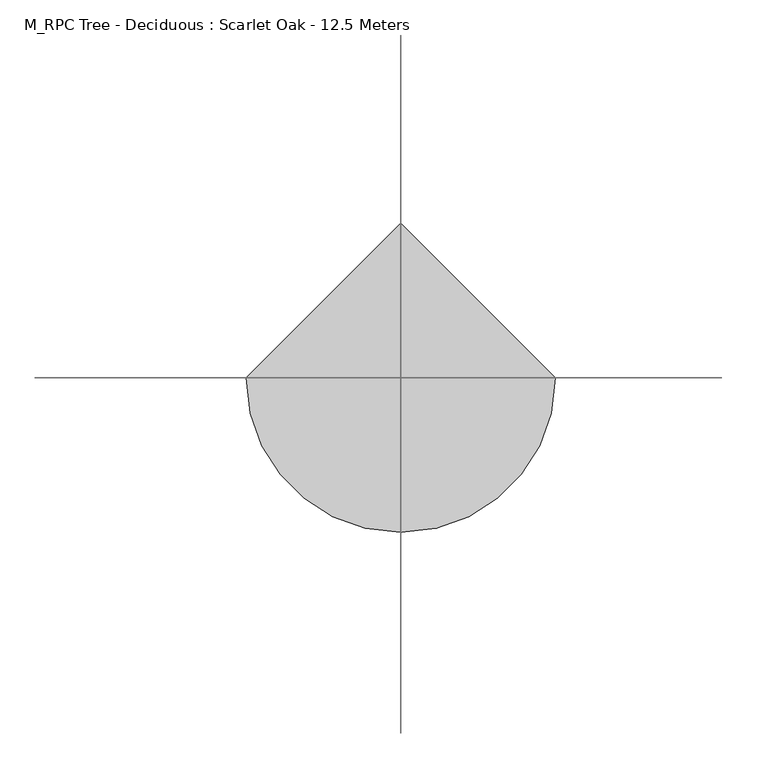
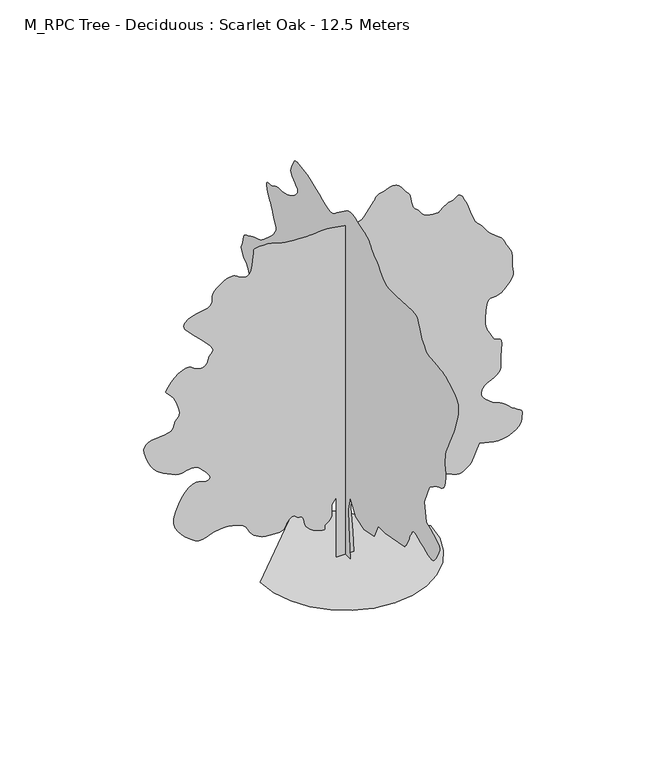
"""IFC4 building model written with IfcOpenShell, lengths in millimetres: geographic element geometry, M_RPC Tree - Deciduous : Scarlet Oak - 12.5 Meters."""

from ifc_helpers import new_model, si_unit, origin, place, context, project, spatial, triangles, source, transform, mapped, element, save


def m_rpc_tree_deciduous_scarlet_oak_12_5_meters_13b38d7d(model_context):
    return source(origin(), model_context, "Body", "Tessellation", [
        triangles([(0.0172504, 306.0074844, 0.0), (0.0172504, -293.5650026, 0.0), (0.0172504, -196.8600042, 1141.1199549), (0.0172504, -177.5184886, 1682.6674953), (0.0172504, -293.5650026, 2185.5349113), (0.0172504, -603.0224945, 1682.6674953), (0.0172504, -1105.8875124, 1527.9400211), (0.0172504, -1686.1174301, 1663.3275421), (0.0172504, -1918.2099495, 2146.8525341), (0.0172504, -2324.3725124, 2146.8525341), (0.0172504, -3446.1498253, 2359.6049549), (0.0172504, -3487.4249222, 2409.394939), (0.0172504, -3527.7000801, 2459.5225479), (0.0172504, -3565.9250725, 2510.3249702), (0.0172504, -3601.0999603, 2562.1500046), (0.0172504, -3632.2248047, 2615.3249565), (0.0172504, -3658.2749588, 2670.2000954), (0.0172504, -3678.2499023, 2727.0748215), (0.0172504, -3697.649881, 2785.6750237), (0.0172504, -3722.1248405, 2845.2748741), (0.0172504, -3750.8248329, 2905.7249634), (0.0172504, -3782.89991, 2966.8500114), (0.0172504, -3817.5248314, 3028.475029), (0.0172504, -3853.8249413, 3090.4500252), (0.0172504, -3890.9999977, 3152.5750122), (0.0172504, -3908.7000801, 3172.6499496), (0.0172504, -3933.1750397, 3188.8498329), (0.0172504, -3971.1750458, 3197.2499016), (0.0172504, -4029.4749756, 3193.9748108), (0.0172504, -4114.8499969, 3175.1500877), (0.0172504, -4234.0499886, 3136.8498093), (0.0172504, -4393.8498276, 3075.2250824), (0.0172504, -4562.5749939, 3002.6998581), (0.0172504, -4706.2499451, 2937.9750298), (0.0172504, -4828.2750549, 2886.4249786), (0.0172504, -4932.0251175, 2853.4999535), (0.0172504, -5020.8999252, 2844.5999153), (0.0172504, -5098.249855, 2865.1248253), (0.0172504, -5167.4996979, 2920.4999336), (0.0172504, -5237.3750839, 3007.7248421), (0.0172504, -5309.5997452, 3113.9000473), (0.0172504, -5377.0996948, 3229.5499649), (0.0172504, -5432.7497864, 3345.1998825), (0.0172504, -5469.4498718, 3451.3750877), (0.0172504, -5480.1248016, 3538.6249947), (0.0172504, -5457.6250122, 3597.424894), (0.0172504, -5402.6498795, 3641.6998077), (0.0172504, -5323.3000717, 3691.0249947), (0.0172504, -5223.6747574, 3744.5999222), (0.0172504, -5107.774855, 3801.5499344), (0.0172504, -4979.7251129, 3861.0500816), (0.0172504, -4843.5499947, 3922.224836), (0.0172504, -4703.3248329, 3984.2498291), (0.0172504, -4587.2749397, 4641.8498062), (0.0172504, -4877.3749649, 5318.7747665), (0.0172504, -4886.5249878, 5331.7001404), (0.0172504, -4900.7247025, 5347.4747589), (0.0172504, -4925.0999588, 5369.0251877), (0.0172504, -4964.6748688, 5399.20009), (0.0172504, -5024.5497025, 5440.8498734), (0.0172504, -5109.8247299, 5496.8999405), (0.0172504, -5225.5246445, 5570.225116), (0.0172504, -5351.0501221, 5636.6501312), (0.0172504, -5462.3497238, 5680.0498077), (0.0172504, -5559.4501923, 5715.3499786), (0.0172504, -5642.3497833, 5757.424736), (0.0172504, -5711.0246613, 5821.1499161), (0.0172504, -5765.4998245, 5921.4001923), (0.0172504, -5805.7496933, 6073.0746552), (0.0172504, -5829.0500153, 6222.0498642), (0.0172504, -5835.7501877, 6317.5748474), (0.0172504, -5830.6249191, 6379.6001312), (0.0172504, -5818.3750854, 6428.1000778), (0.0172504, -5803.7748138, 6483.0246323), (0.0172504, -5791.5499786, 6564.3249023), (0.0172504, -5786.4247101, 6691.9996674), (0.0172504, -5788.2251816, 6832.849791), (0.0172504, -5796.1246994, 6949.6746368), (0.0172504, -5813.8247818, 7056.3751007), (0.0172504, -5845.0496201, 7166.7747574), (0.0172504, -5893.550148, 7294.7750839), (0.0172504, -5963.0249771, 7454.2496521), (0.0172504, -6057.1750443, 7659.049942), (0.0172504, -6146.5748199, 7844.1746887), (0.0172504, -6206.1746704, 7955.8748474), (0.0172504, -6246.4751175, 8024.9497009), (0.0172504, -6277.9999374, 8082.1746964), (0.0172504, -6311.2246536, 8158.3496979), (0.0172504, -6356.599791, 8284.2751511), (0.0172504, -6424.6747055, 8490.6997604), (0.0172504, -6498.0248795, 8729.4997192), (0.0172504, -6547.3747742, 8935.1499573), (0.0172504, -6565.2498459, 9112.3746048), (0.0172504, -6544.199968, 9265.925116), (0.0172504, -6476.8250107, 9400.5250397), (0.0172504, -6355.6498489, 9520.8996689), (0.0172504, -6173.2249374, 9631.8248749), (0.0172504, -5996.2246948, 9723.0001236), (0.0172504, -5879.7998245, 9785.7747803), (0.0172504, -5799.2250916, 9827.2001587), (0.0172504, -5729.799678, 9854.4496582), (0.0172504, -5646.85009, 9874.575174), (0.0172504, -5525.6749283, 9894.699527), (0.0172504, -5341.575119, 9921.9501892), (0.0172504, -5144.0999634, 9943.4244598), (0.0172504, -4990.9500092, 9951.725116), (0.0172504, -4869.5998581, 9962.0244873), (0.0172504, -4767.5499825, 9989.5995483), (0.0172504, -4672.2499855, 10049.6493713), (0.0172504, -4571.2000488, 10157.425351), (0.0172504, -4451.8750648, 10328.0998169), (0.0172504, -4347.6750298, 10515.7499908), (0.0172504, -4286.1000092, 10666.5500885), (0.0172504, -4245.8498497, 10783.8243256), (0.0172504, -4205.5749825, 10871.0003998), (0.0172504, -4143.9999619, 10931.4501984), (0.0172504, -4039.7999268, 10968.5502594), (0.0172504, -3871.650016, 10985.7003754), (0.0172504, -2943.2749969, 10927.6748474), (0.0172504, -2772.1499771, 10930.6746643), (0.0172504, -2632.8250511, 10930.2746887), (0.0172504, -2514.4500092, 10937.3242584), (0.0172504, -2406.244986, 10962.6250397), (0.0172504, -2297.3599171, 11017.0496246), (0.0172504, -2176.9724979, 11111.3752625), (0.0172504, -2034.2549011, 11256.4745453), (0.0172504, -1896.7275398, 11403.0249023), (0.0172504, -1793.7049038, 11502.8746216), (0.0172504, -1717.0749882, 11568.5752625), (0.0172504, -1658.7124168, 11612.6248993), (0.0172504, -1610.5024235, 11647.5250946), (0.0172504, -1564.3199226, 11685.7995026), (0.0172504, -1512.0500027, 11739.9996826), (0.0172504, -1461.8649845, 11803.9992645), (0.0172504, -1420.8125484, 11863.6002777), (0.0172504, -1379.087479, 11919.1503754), (0.0172504, -1326.8724976, 11970.9495392), (0.0172504, -1254.3574471, 12019.4000702), (0.0172504, -1151.7299904, 12064.7996246), (0.0172504, -1009.182514, 12107.4749268), (0.0172504, -849.1549999, 12154.4999634), (0.0172504, -699.9524792, 12206.6002716), (0.0172504, -560.5600064, 12254.6496643), (0.0172504, -429.9675053, 12289.4998627), (0.0172504, -307.1549798, 12302.0246796), (0.0172504, -191.1079934, 12283.0746735), (0.0172504, -80.8134993, 12223.5248199), (0.0172504, 499.4174812, 11798.0252106), (0.0172504, 562.2325061, 11740.8496307), (0.0172504, 623.0199657, 11688.7493225), (0.0172504, 689.217524, 11646.7751404), (0.0172504, 768.2749804, 11620.0500275), (0.0172504, 867.6299623, 11613.6248383), (0.0172504, 994.7275097, 11632.5748444), (0.0172504, 1157.0125168, 11681.9753174), (0.0172504, 1341.1749676, 11755.3243286), (0.0172504, 1526.6899521, 11837.8251068), (0.0172504, 1710.1749733, 11922.0246185), (0.0172504, 1888.2475342, 12000.4500641), (0.0172504, 2057.5249924, 12065.6995697), (0.0172504, 2214.6199093, 12110.3003357), (0.0172504, 2356.1550201, 12126.8249084), (0.0172504, 2484.8875694, 12135.849939), (0.0172504, 2604.4750374, 12156.3742676), (0.0172504, 2712.9248131, 12178.575238), (0.0172504, 2808.1498146, 12192.6743774), (0.0172504, 2888.1748718, 12188.8501923), (0.0172504, 2950.9248207, 12157.2753754), (0.0172504, 2994.400074, 12088.1249451), (0.0172504, 3033.2500282, 12001.2500153), (0.0172504, 3077.8499222, 11921.1246735), (0.0172504, 3119.7499809, 11845.0502472), (0.0172504, 3150.4998482, 11770.3245758), (0.0172504, 3161.6000427, 11694.2745667), (0.0172504, 3144.6249161, 11614.1503876), (0.0172504, 3091.124984, 11527.2498779), (0.0172504, 3009.2500397, 11447.6245056), (0.0172504, 2921.5998665, 11385.2492432), (0.0172504, 2841.4248184, 11331.3502075), (0.0172504, 2781.8749649, 11277.1000305), (0.0172504, 2756.1750801, 11213.7248291), (0.0172504, 2777.4749428, 11132.4251404), (0.0172504, 2859.0249069, 11024.3747589), (0.0172504, 2971.6250107, 10916.724353), (0.0172504, 3077.7999252, 10838.2000763), (0.0172504, 3178.2249001, 10782.3), (0.0172504, 3273.574894, 10742.6745117), (0.0172504, 3364.5248657, 10712.8251709), (0.0172504, 3451.7750633, 10686.4000397), (0.0172504, 3535.9498672, 10656.8995148), (0.0172504, 3620.024968, 10634.1753204), (0.0172504, 3706.4749237, 10626.6746155), (0.0172504, 3795.2750267, 10625.9502411), (0.0172504, 3886.4499847, 10623.5248077), (0.0172504, 3979.9997978, 10610.9499939), (0.0172504, 4075.9250473, 10579.7495728), (0.0172504, 4174.1998627, 10521.5252197), (0.0172504, 4275.775058, 10469.7993073), (0.0172504, 4375.6250679, 10451.2492767), (0.0172504, 4464.9998451, 10446.8995422), (0.0172504, 4535.0999268, 10437.8245148), (0.0172504, 4577.0999794, 10405.075351), (0.0172504, 4582.2249573, 10329.6753021), (0.0172504, 4541.6998146, 10192.7243591), (0.0172504, 4481.7999825, 10048.5994354), (0.0172504, 4432.0748199, 9951.4995483), (0.0172504, 4388.424868, 9882.1247131), (0.0172504, 4346.824791, 9821.224942), (0.0172504, 4303.174839, 9749.4996689), (0.0172504, 4253.4249687, 9647.6750702), (0.0172504, 4193.5498444, 9496.4499985), (0.0172504, 4130.2749275, 9347.6997757), (0.0172504, 4075.8250534, 9253.7496964), (0.0172504, 4034.1999779, 9195.999733), (0.0172504, 4009.500032, 9155.8498581), (0.0172504, 4005.7749687, 9114.7000443), (0.0172504, 4027.0998299, 9053.8996857), (0.0172504, 4077.4999512, 8954.8999146), (0.0172504, 4167.2249977, 8823.6747849), (0.0172504, 4293.1248711, 8684.3501495), (0.0172504, 4439.3499573, 8545.349913), (0.0172504, 4589.9500671, 8415.1497208), (0.0172504, 4729.0750053, 8302.1996384), (0.0172504, 4840.7748734, 8214.9747299), (0.0172504, 4909.1747681, 8161.9000626), (0.0172504, 4969.9001312, 8128.6997635), (0.0172504, 5061.0747986, 8095.1500671), (0.0172504, 5170.5250946, 8060.9248306), (0.0172504, 5286.0750183, 8025.6746567), (0.0172504, 5395.524733, 7989.0751465), (0.0172504, 5486.6999817, 7950.8001572), (0.0172504, 5547.4247635, 7910.4747116), (0.0172504, 5598.275148, 7876.9750122), (0.0172504, 5663.0246841, 7853.2997131), (0.0172504, 5734.1749924, 7830.2999542), (0.0172504, 5804.3247803, 7798.8251312), (0.0172504, 5866.0250839, 7749.7746368), (0.0172504, 5911.8001968, 7673.9746124), (0.0172504, 5934.2499893, 7562.325032), (0.0172504, 5952.6250305, 7450.1749008), (0.0172504, 5984.1998474, 7370.8500916), (0.0172504, 6018.4750809, 7312.1496048), (0.0172504, 6044.9996246, 7261.899765), (0.0172504, 6053.224704, 7207.9501511), (0.0172504, 6032.699794, 7138.074765), (0.0172504, 5972.9249542, 7040.1249298), (0.0172504, 5898.7248322, 6948.3747162), (0.0172504, 5838.7250061, 6893.5251572), (0.0172504, 5788.2001831, 6857.9500031), (0.0172504, 5742.4000717, 6824.0497467), (0.0172504, 5696.6249588, 6774.2498795), (0.0172504, 5646.1001358, 6690.9747299), (0.0172504, 5586.0997284, 6556.5997925), (0.0172504, 5520.6996506, 6421.9998688), (0.0172504, 5460.6998245, 6337.1498154), (0.0172504, 5411.5249191, 6283.0746277), (0.0172504, 5378.6001846, 6240.824881), (0.0172504, 5367.3247101, 6191.4999847), (0.0172504, 5383.09991, 6116.0999359), (0.0172504, 5431.3748703, 5995.7247253), (0.0172504, 5495.5000259, 5864.0496231), (0.0172504, 5555.8748291, 5761.8250488), (0.0172504, 5613.5747955, 5680.5747757), (0.0172504, 5669.5498672, 5611.8249023), (0.0172504, 5724.8749786, 5547.1497803), (0.0172504, 5780.5250702, 5478.0749268), (0.0172504, 5837.5250793, 5396.1496948), (0.0172504, 5903.6751114, 5315.3499756), (0.0172504, 5980.6500641, 5249.4249298), (0.0172504, 6060.324852, 5189.6000931), (0.0172504, 6134.5999695, 5127.0498413), (0.0172504, 6195.3247513, 5053.0247086), (0.0172504, 6234.3996918, 4958.6746536), (0.0172504, 6243.6997055, 4835.2499199), (0.0172504, 6251.5248093, 4738.3250221), (0.0172504, 6280.349794, 4706.349939), (0.0172504, 6313.2251129, 4704.825032), (0.0172504, 6333.2500534, 4699.249791), (0.0172504, 6323.4750687, 4655.0998695), (0.0172504, 6267.0500244, 4537.8750481), (0.0172504, 6146.999794, 4313.0498177), (0.0172504, 6021.4748978, 4060.8748032), (0.0172504, 5945.6998718, 3875.3750793), (0.0172504, 5898.3248566, 3742.6250427), (0.0172504, 5858.0749878, 3648.7999557), (0.0172504, 5803.5998245, 3580.0000854), (0.0172504, 5713.6000854, 3522.3748238), (0.0172504, 5566.7747452, 3462.0500175), (0.0172504, 5397.2496277, 3413.0998077), (0.0172504, 5248.0500137, 3392.5748978), (0.0172504, 5111.0246567, 3390.9999939), (0.0172504, 4978.0746323, 3398.8998024), (0.0172504, 4841.0498566, 3406.7749031), (0.0172504, 4691.8499519, 3405.1999992), (0.0172504, 4522.3498329, 3384.6750893), (0.0172504, 4353.2999771, 3366.3000481), (0.0172504, 4207.2498802, 3370.249807), (0.0172504, 4078.7998718, 3385.7000267), (0.0172504, 3962.5249924, 3401.8249146), (0.0172504, 3853.0249901, 3407.7998405), (0.0172504, 3744.8749054, 3392.799884), (0.0172504, 3632.6500694, 3345.9998337), (0.0172504, 3525.249939, 3296.2499634), (0.0172504, 3436.4248375, 3270.1998093), (0.0172504, 3368.249929, 3253.6249489), (0.0172504, 3322.75009, 3232.3250862), (0.0172504, 3301.9499062, 3192.0499283), (0.0172504, 3307.8748352, 3118.6500481), (0.0172504, 3342.5500443, 2997.8498634), (0.0172504, 3398.4748283, 2869.5248474), (0.0172504, 3465.5748024, 2778.7248665), (0.0172504, 3542.0000793, 2719.2500084), (0.0172504, 3625.8499031, 2684.8000763), (0.0172504, 3715.274968, 2669.1248703), (0.0172504, 3808.4248055, 2665.9500641), (0.0172504, 3903.4248207, 2669.0498749), (0.0172504, 4270.9250633, 2262.8999565), (0.0172504, 4299.7250496, 2217.1674282), (0.0172504, 4327.3498169, 2170.5925095), (0.0172504, 4352.6250183, 2122.3249615), (0.0172504, 4374.3248566, 2071.5174522), (0.0172504, 4391.2999832, 2017.3299168), (0.0172504, 4402.3498901, 1958.9124069), (0.0172504, 4406.2999397, 1895.4199162), (0.0172504, 4405.6249809, 1829.2200325), (0.0172504, 4400.8999786, 1763.6974331), (0.0172504, 4388.0248924, 1699.5299835), (0.0172504, 4362.9999664, 1637.3900265), (0.0172504, 4321.7248695, 1577.9574623), (0.0172504, 4260.1498489, 1521.9075405), (0.0172504, 4174.1998627, 1469.9175453), (0.0172504, 4092.2249245, 1425.7650078), (0.0172504, 4034.5999535, 1391.4249527), (0.0172504, 3985.4250481, 1364.8674168), (0.0172504, 3928.800016, 1344.0599659), (0.0172504, 3848.8499542, 1326.9749622), (0.0172504, 3729.6499626, 1311.5799717), (0.0172504, 3555.2998489, 1295.8475018), (0.0172504, 3356.9750359, 1298.1024513), (0.0172504, 3174.2248535, 1332.8375404), (0.0172504, 3003.6500908, 1392.27243), (0.0172504, 2841.8750816, 1468.6199501), (0.0172504, 2685.525032, 1554.1049938), (0.0172504, 2531.1748604, 1640.9424259), (0.0172504, 2375.4949734, 1721.3500179), (0.0172504, 2236.6674007, 1794.4849434), (0.0172504, 2129.3049133, 1863.5599422), (0.0172504, 2044.6099377, 1926.8850014), (0.0172504, 1973.7875164, 1982.7650208), (0.0172504, 1908.0399307, 2029.5099873), (0.0172504, 1838.5700432, 2065.4300331), (0.0172504, 1756.5824604, 2088.8299129), (0.0172504, 1666.4174698, 2108.5649002), (0.0172504, 1577.6074837, 2133.0375343), (0.0172504, 1489.134977, 2159.8799366), (0.0172504, 1399.9875114, 2186.7200134), (0.0172504, 1309.1449459, 2211.1925022), (0.0172504, 1215.5974583, 2230.9274895), (0.0172504, 1118.3299942, 2243.5575325), (0.0172504, 1018.8625191, 2250.1549496), (0.0172504, 919.3925005, 2253.7074944), (0.0172504, 819.9249527, 2254.7224033), (0.0172504, 720.4574776, 2253.7074944), (0.0172504, 620.9900024, 2251.1700039), (0.0172504, 521.5199839, 2247.6174591), (0.0172504, 422.0525087, 2243.5575325), (0.0172504, 228.6430025, 1953.4425373), (0.0172504, 189.960498, 1508.5999226), (280.4450004, 0.0006008, 0.0092122), (-299.78499, 0.0006008, 0.0092122), (-299.78499, 0.0004756, 2127.5199932), (-454.5149895, 0.0004756, 1914.7698978), (-454.5149895, 0.0005007, 1682.6775238), (-450.962481, 0.0005007, 1628.8274677), (-450.962481, 0.0005007, 1575.1449886), (-458.0674979, 0.0005007, 1521.8024597), (-475.8274967, 0.0005257, 1468.967458), (-507.8000001, 0.0005257, 1416.8100311), (-557.5350094, 0.0005257, 1365.4949947), (-628.5824896, 0.0005257, 1315.1974834), (-684.2375227, 0.0005257, 1262.982502), (-699.6325132, 0.0005257, 1210.0899456), (-696.0799685, 0.0005257, 1162.9524885), (-694.8950117, 0.0005257, 1127.990015), (-717.3950191, 0.0005257, 1111.6374521), (-784.8899546, 0.0005257, 1120.3224598), (-918.6974848, 0.0005257, 1160.4700092), (-1071.3399845, 0.0005257, 1223.0050003), (-1185.4124548, 0.0005257, 1293.6575191), (-1267.3424103, 0.0005257, 1371.0799736), (-1323.5625252, 0.0005257, 1453.9124176), (-1360.49748, 0.0005007, 1540.8049335), (-1384.5749348, 0.0005007, 1630.4049877), (-1402.2250202, 0.0005007, 1721.359901), (-1406.7349194, 0.0005007, 1746.1124599), (-1413.4449749, 0.0005007, 1770.1899147), (-1424.5524364, 0.0005007, 1792.9174519), (-1442.2599312, 0.0005007, 1813.6099388), (-1468.7599125, 0.0005007, 1831.5975037), (-1506.2599491, 0.0005007, 1846.2024261), (-1556.9524944, 0.0005007, 1856.747422), (-1607.6450397, 0.0005007, 1874.1124958), (-1647.509903, 0.0005007, 1903.3224861), (-1682.3024014, 0.0004756, 1934.8999191), (-1717.7700039, 0.0004756, 1959.3724079), (-1759.6674465, 0.0004756, 1967.2674202), (-1813.7424889, 0.0004756, 1949.1099529), (-1885.7500122, 0.0005007, 1895.4274738), (-1949.0724552, 0.0005007, 1820.3199944), (-1984.9925011, 0.0005007, 1746.902528), (-2011.0999191, 0.0005007, 1679.2374722), (-2044.9875309, 0.0005007, 1621.382428), (-2104.2525181, 0.0005007, 1577.402409), (-2206.4824699, 0.0005007, 1551.3499294), (-2369.2750042, 0.0005007, 1547.2900028), (-2549.149926, 0.0005007, 1559.2449417), (-2695.2000229, 0.0005007, 1578.979929), (-2813.8250496, 0.0005007, 1607.1750103), (-2911.4999016, 0.0005007, 1644.5025284), (-2994.6250603, 0.0005007, 1691.6425289), (-3069.5998444, 0.0005007, 1749.2724415), (-3142.9250198, 0.0005007, 1818.0648994), (-3205.1000038, 0.0005007, 1893.5100037), (-3249.7248962, 0.0004756, 1969.2975288), (-3287.549913, 0.0004756, 2043.389954), (-3329.4499718, 0.0004756, 2113.7624027), (-3386.2249947, 0.0004756, 2178.3824409), (-3468.7249008, 0.0004756, 2235.2224308), (-3587.7499031, 0.0004756, 2282.2499382), (-3707.4248657, 0.0004756, 2317.9974655), (-3794.2497986, 0.0004506, 2343.2600224), (-3862.8249733, 0.0004506, 2359.3875263), (-3927.674794, 0.0004506, 2367.7325111), (-4003.3248276, 0.0004506, 2369.6499813), (-4104.3750549, 0.0004506, 2366.4924706), (-4245.3498802, 0.0004506, 2359.6125126), (-4400.3500122, 0.0004506, 2335.1974331), (-4538.1250328, 0.0004756, 2289.8050003), (-4665.0498436, 0.0004756, 2240.3524956), (-4787.5749229, 0.0004756, 2203.7574909), (-4912.1501678, 0.0004756, 2196.9349422), (-5045.1501892, 0.0004756, 2236.7999508), (-5193.0498825, 0.0004506, 2340.272414), (-5347.7997391, 0.0004506, 2478.6475433), (-5490.6747391, 0.0004506, 2615.9999153), (-5612.2498764, 0.0004256, 2758.4499413), (-5703.0251495, 0.0004256, 2912.049868), (-5753.5499725, 0.0004256, 3082.8999046), (-5754.3499237, 0.0004005, 3277.0999695), (-5695.9250015, 0.0004005, 3500.7249825), (-5598.1501556, 0.0003755, 3726.2748779), (-5489.1998291, 0.0003755, 3919.6999901), (-5372.1499969, 0.0003505, 4077.2499664), (-5250.0248932, 0.0003505, 4195.2000343), (-5125.8499146, 0.0003505, 4269.8498383), (-5002.6998734, 0.0003505, 4297.4998947), (-4883.6001663, 0.0003505, 4274.3748528), (-4771.2750458, 0.0003505, 4235.4749016), (-4671.8250114, 0.0003505, 4218.8750427), (-4593.3248611, 0.0003505, 4225.6499199), (-4543.9249695, 0.0003505, 4256.7750549), (-4531.7498405, 0.0003505, 4313.2748039), (-4564.899852, 0.0003505, 4396.1749763), (-4651.4997986, 0.0003254, 4506.4749298), (-4752.500029, 0.0003254, 4617.0998634), (-4829.4749817, 0.0003254, 4702.3498924), (-4891.5496811, 0.0003254, 4765.2748306), (-4947.8747314, 0.0003254, 4808.9247826), (-5007.6001556, 0.0003254, 4836.3248543), (-5079.8248169, 0.0003004, 4850.5498581), (-5173.7248993, 0.0003004, 4854.5999016), (-5270.0248352, 0.0003254, 4845.5248741), (-5349.7751999, 0.0003254, 4824.5999886), (-5422.3998367, 0.0003254, 4801.3249557), (-5497.39991, 0.0003254, 4785.1247818), (-5584.2248428, 0.0003254, 4785.5250481), (-5692.3746368, 0.0003254, 4811.9748871), (-5831.3248764, 0.0003004, 4873.9498833), (-5978.7751785, 0.0003004, 4948.0997177), (-6108.6248108, 0.0003004, 5012.4248611), (-6224.624707, 0.0003004, 5078.4748993), (-6330.4496429, 0.0003004, 5157.6997147), (-6429.8749695, 0.0003004, 5261.5997681), (-6526.574881, 0.0002754, 5401.7249359), (-6624.2997299, 0.0002754, 5589.5750977), (-6705.1000305, 0.0002503, 5784.4998276), (-6749.6996338, 0.0002503, 5941.2001465), (-6759.8001801, 0.0002503, 6064.0746231), (-6737.074823, 0.0002253, 6157.4997345), (-6683.2246216, 0.0002253, 6225.8996292), (-6599.9500534, 0.0002253, 6273.6496216), (-6488.899855, 0.0002253, 6305.1750229), (-6357.7997177, 0.0002253, 6323.2750809), (-6219.2750336, 0.0002253, 6333.9500107), (-6082.3996674, 0.0002253, 6346.2748398), (-5956.3748016, 0.0002253, 6369.4501694), (-5850.3248795, 0.0002253, 6412.5998611), (-5773.3499268, 0.0002253, 6484.8251038), (-5734.5999664, 0.0002003, 6595.2997559), (-5705.9749695, 0.0002003, 6701.9746399), (-5661.749762, 0.0002003, 6771.4500504), (-5614.8497177, 0.0002003, 6825.699646), (-5578.0746368, 0.0002003, 6886.6999924), (-5564.3248947, 0.0001752, 6976.4747452), (-5586.4247086, 0.0001752, 7116.9998886), (-5657.2500366, 0.0001752, 7330.2496628), (-5757.5497284, 0.0001502, 7540.2996323), (-5853.4746872, 0.0001502, 7672.5247009), (-5935.8498917, 0.0001502, 7750.975145), (-5995.5747345, 0.0001252, 7799.6250824), (-6023.4747757, 0.0001252, 7842.5247894), (-6010.4499893, 0.0001252, 7903.7251236), (-5947.3497711, 0.0001252, 8007.1996216), (-5845.6501648, 0.0001252, 8136.3248795), (-5728.0247864, 0.0001001, 8253.9496765), (-5602.2749039, 0.0001001, 8353.3000076), (-5476.1750427, 0.0001001, 8427.6251221), (-5357.5497253, 0.0001001, 8470.1248535), (-5254.1246429, 0.0001001, 8474.0746124), (-5173.7248993, 0.0001001, 8432.6998123), (-5094.9000595, 0.0001001, 8371.00009), (-4997.8001724, 0.0001001, 8322.8501221), (-4892.5751999, 0.0001001, 8294.6500992), (-4789.3748131, 0.0001001, 8292.8496277), (-4698.3748444, 0.0001001, 8323.8750595), (-4629.6999664, 0.0001001, 8394.1248413), (-4593.4998505, 0.0001001, 8510.0497421), (-4560.3248405, 0.0001001, 8620.5749725), (-4508.224823, 7.51e-05, 8686.1000427), (-4458.4999512, 7.51e-05, 8730.2996704), (-4432.4497971, 7.51e-05, 8776.8747345), (-4451.3998032, 7.51e-05, 8849.4999527), (-4536.6498322, 7.51e-05, 8971.8750412), (-4709.5500343, 5.01e-05, 9167.6497192), (-4926.3498825, 5.01e-05, 9388.7995926), (-5120.1496811, 2.5e-05, 9575.0998489), (-5277.4249649, 2.5e-05, 9731.9745758), (-5384.5998184, 2.5e-05, 9864.8246063), (-5428.2000641, 0.0, 9979.0746094), (-5394.6497864, 0.0, 10080.1254181), (-5270.4248108, 0.0, 10173.3743774), (-5104.7500397, 0.0, 10245.2246429), (-4956.3497955, 0.0, 10286.2744629), (-4825.8749107, 0.0, 10308.3742767), (-4714.0000534, -2.5e-05, 10323.3745239), (-4621.3998917, -2.5e-05, 10343.1000641), (-4548.7749641, -2.5e-05, 10379.4245911), (-4496.7749405, -2.5e-05, 10444.1497101), (-4470.8500694, -2.5e-05, 10520.7252686), (-4466.9000198, -2.5e-05, 10587.8246613), (-4471.4000359, -2.5e-05, 10650.1999237), (-4470.8500694, -2.5e-05, 10712.5751862), (-4451.6747864, -5.01e-05, 10779.6745789), (-4400.3500122, -5.01e-05, 10856.2501373), (-4303.3748268, -5.01e-05, 10947.0248291), (-4184.6748047, -5.01e-05, 11036.8495789), (-4076.1250351, -5.01e-05, 11106.7243835), (-3976.0500389, -7.51e-05, 11155.5993073), (-3882.7249214, -7.51e-05, 11182.4999908), (-3794.4750755, -7.51e-05, 11186.3997528), (-3709.6000237, -7.51e-05, 11166.2498199), (-3626.4498665, -5.01e-05, 11121.1002502), (-3540.7248665, -5.01e-05, 11065.9001312), (-3452.3250298, -5.01e-05, 11022.8748505), (-3365.6000908, -5.01e-05, 11001.8249725), (-3284.9500717, -5.01e-05, 11012.5998962), (-3214.7999931, -5.01e-05, 11064.9746063), (-3159.5498772, -7.51e-05, 11168.7996643), (-3123.5750381, -7.51e-05, 11333.8500549), (-3102.0998955, -7.51e-05, 11511.0752838), (-3086.6999634, -0.0001001, 11648.0250641), (-3076.3750122, -0.0001001, 11749.4746857), (-3070.1248123, -0.0001001, 11820.1250244), (-3066.9000092, -0.0001001, 11864.7246277), (-3065.7250809, -0.0001001, 11888.0243683), (-3065.5500916, -0.0001001, 11894.7251221), (-3040.1248993, -0.0001001, 11898.674881), (-2971.0500458, -0.0001001, 11907.37435), (-2869.1498703, -0.0001001, 11916.0494019), (-2745.2748734, -0.0001001, 11920.0003235), (-2610.2249771, -0.0001001, 11914.4750793), (-2474.8323692, -0.0001001, 11894.7251221), (-2349.9349056, -0.0001001, 11856.0495758), (-2235.4099194, -0.0001001, 11813.024295), (-2120.5474537, -0.0001001, 11781.8494537), (-2000.2725277, -0.0001001, 11760.1251984), (-1869.507399, -0.0001001, 11745.5249268), (-1723.1824642, -0.0001001, 11735.6743652), (-1556.2175102, -0.0001001, 11728.174823), (-1363.5400269, -0.0001001, 11720.6752808), (-1177.5749971, -0.0001001, 11719.599765), (-1024.4249702, -0.0001001, 11728.6747925), (-889.5449764, -0.0001001, 11741.475174), (-758.3875025, -0.0001001, 11751.5745575), (-616.4049625, -0.0001001, 11752.5244995), (-449.0450109, -0.0001001, 11737.9253906), (-241.7632409, -0.0001001, 11701.3252991), (-32.2257492, -0.0001001, 11657.8000488), (136.7124946, -0.0001001, 11627.7995544), (271.8174929, -0.0001001, 11613.0248749), (379.8574825, -0.0001001, 11615.1503265), (467.5974758, -0.0001001, 11635.9246399), (541.8025031, -0.0001001, 11676.9744598), (609.2425, -0.0001001, 11739.9996826), (899.3574589, -0.0001252, 12107.4749268), (942.8899761, -0.0001252, 12164.1493744), (977.6249926, -0.0001252, 12217.4496094), (1008.9749685, -0.0001252, 12266.3245331), (1042.3574512, -0.0001252, 12309.7997864), (1083.1825029, -0.0001252, 12346.8498505), (1136.864982, -0.0001252, 12376.4503693), (1208.8149508, -0.0001252, 12397.6002411), (1297.0049892, -0.0001502, 12421.8499237), (1393.3149536, -0.0001502, 12454.2246918), (1494.0224693, -0.0001502, 12483.8752075), (1595.4100307, -0.0001502, 12499.9998047), (1693.7499584, -0.0001502, 12491.7747253), (1785.3224213, -0.0001502, 12448.349469), (1866.4099136, -0.0001252, 12358.9246948), (1938.4149662, -0.0001252, 12256.9251068), (2004.3324543, -0.0001252, 12177.5752991), (2062.8075188, -0.0001252, 12112.7746033), (2112.4850098, -0.0001252, 12054.4246765), (2152.0125389, -0.0001252, 11994.3748535), (2180.0374271, -0.0001001, 11924.5000488), (2195.2049606, -0.0001001, 11836.6995941), (2205.7499565, -0.0001001, 11745.6993347), (2220.3550243, -0.0001001, 11669.9248901), (2238.3424438, -0.0001001, 11606.8252533), (2259.0349308, -7.51e-05, 11553.8749969), (2281.7599972, -7.51e-05, 11508.5242767), (2305.8374519, -7.51e-05, 11468.274408), (2330.5924816, -7.51e-05, 11430.5499664), (2355.6274361, -7.51e-05, 11413.5742584), (2381.6799156, -7.51e-05, 11394.2242767), (2409.760033, -7.51e-05, 11370.1501648), (2440.8873482, -7.51e-05, 11338.9753235), (2476.0724098, -7.51e-05, 11298.3243164), (2516.3248947, -7.51e-05, 11245.8251953), (2562.6749725, -7.51e-05, 11179.1246155), (2631.3748489, -5.01e-05, 11115.7249969), (2728.4750267, -5.01e-05, 11072.3253204), (2839.7749191, -5.01e-05, 11045.1246552), (2951.0748116, -5.01e-05, 11030.4743866), (3048.1749893, -5.01e-05, 11024.6003265), (3116.8748657, -5.01e-05, 11023.8247925), (3142.9250198, -5.01e-05, 11024.4003387), (3156.2750771, -5.01e-05, 11038.3250702), (3192.9998703, -5.01e-05, 11074.2252045), (3247.9750031, -5.01e-05, 11123.3501129), (3316.1499115, -7.51e-05, 11176.8503357), (3392.4249069, -7.51e-05, 11225.9752441), (3471.7750053, -7.51e-05, 11261.8997955), (3549.0749382, -7.51e-05, 11275.824527), (3618.3750687, -7.51e-05, 11292.800235), (3679.549823, -7.51e-05, 11331.0746429), (3736.3498444, -7.51e-05, 11371.7244873), (3792.4499084, -7.51e-05, 11395.8253418), (3851.6000771, -7.51e-05, 11384.3748779), (3917.5248322, -7.51e-05, 11318.4498322), (3993.9248199, -7.51e-05, 11179.1246155), (4065.8750793, -5.01e-05, 11015.4253052), (4119.5500008, -5.01e-05, 10883.1996552), (4160.3748344, -5.01e-05, 10773.6249481), (4193.7498322, -2.5e-05, 10677.9493927), (4225.0999535, -2.5e-05, 10587.3246918), (4259.8498672, -2.5e-05, 10493.0002167), (4303.3748268, -2.5e-05, 10386.1253448), (4348.1000038, 0.0, 10292.3496735), (4386.3749931, 0.0, 10232.749823), (4423.6500435, 0.0, 10191.7744171), (4465.3248253, 0.0, 10153.824408), (4516.799881, 0.0, 10103.3495819), (4583.4998795, 0.0, 10024.7997253), (4670.850071, 0.0, 9902.6002075), (4778.3749031, 2.5e-05, 9766.6003693), (4896.3999664, 2.5e-05, 9652.9247498), (5016.4501968, 2.5e-05, 9555.474884), (5130.0746567, 5.01e-05, 9468.1999786), (5228.8000259, 5.01e-05, 9384.974826), (5304.2000748, 5.01e-05, 9299.6997986), (5347.7997391, 5.01e-05, 9206.3246841), (5382.0249756, 5.01e-05, 9114.7500412), (5429.774968, 7.51e-05, 9032.6498199), (5483.3001892, 7.51e-05, 8950.5495987), (5534.7749542, 7.51e-05, 8858.9749557), (5576.449736, 7.51e-05, 8748.4747238), (5600.5250107, 0.0001001, 8609.5250656), (5599.22509, 0.0001001, 8432.6998123), (5596.5746704, 0.0001001, 8262.7497208), (5611.174942, 0.0001252, 8138.7997284), (5627.1251312, 0.0001252, 8042.949765), (5628.5500443, 0.0001252, 7957.224765), (5599.5000732, 0.0001252, 7863.7496567), (5524.1250229, 0.0001502, 7744.5249573), (5386.474704, 0.0001502, 7581.6750137), (5223.124791, 0.0001502, 7444.9496384), (5081.4247192, 0.0001502, 7390.0750809), (4961.7000504, 0.0001502, 7378.1746445), (4864.3248894, 0.0001502, 7370.3501221), (4789.5997993, 0.0001752, 7327.6498215), (4737.9000481, 0.0001752, 7211.2249512), (4709.5250359, 0.0001752, 6982.1249817), (4698.9248108, 0.0002003, 6728.5997589), (4700.5250038, 0.0002003, 6550.1751846), (4714.6000168, 0.0002253, 6424.8996918), (4741.5748238, 0.0002253, 6330.7246262), (4781.7249893, 0.0002253, 6245.7001648), (4835.3999107, 0.0002253, 6147.7997452), (4902.950148, 0.0002503, 6015.074707), (4980.0250946, 0.0002503, 5899.6497757), (5057.7999985, 0.0002503, 5847.1500732), (5129.7996735, 0.0002503, 5825.7746338), (5189.6250916, 0.0002503, 5803.7248169), (5230.8499008, 0.0002503, 5749.1996567), (5247.0250763, 0.0002754, 5630.3749329), (5231.7498459, 0.0002754, 5415.4996765), (5210.9999496, 0.0003004, 5178.6001831), (5207.8251434, 0.0003004, 5005.3247131), (5211.4499222, 0.0003004, 4881.0997375), (5210.9999496, 0.0003254, 4791.3999802), (5195.6497238, 0.0003254, 4721.6498772), (5154.5999039, 0.0003254, 4657.3000259), (5077.0249878, 0.0003254, 4583.8248596), (4983.2998947, 0.0003254, 4514.9249954), (4900.3997223, 0.0003254, 4468.3499313), (4827.3248222, 0.0003254, 4435.6498924), (4763.0499664, 0.0003505, 4408.3498146), (4706.5499268, 0.0003505, 4378.0249214), (4656.8250549, 0.0003505, 4336.1748596), (4612.8248337, 0.0003505, 4274.3748528), (4577.8749321, 0.0003505, 4202.8248596), (4558.1249748, 0.0003505, 4135.32491), (4557.0000435, 0.0003505, 4068.8498978), (4577.8749321, 0.0003755, 4000.3250107), (4624.1000175, 0.0003755, 3926.7498505), (4699.0998001, 0.0003755, 3845.024897), (4806.2499458, 0.0003755, 3752.1750412), (4919.7997009, 0.0003755, 3670.8000664), (5016.1246353, 0.0003755, 3617.4998314), (5101.5996506, 0.0004005, 3580.1250778), (5182.6999329, 0.0004005, 3546.4748062), (5265.8000931, 0.0004005, 3504.3500519), (5357.374736, 0.0004005, 3441.5748138), (5463.8246338, 0.0004005, 3345.9998337), (5576.8497116, 0.0004005, 3247.2750458), (5681.0497467, 0.0004005, 3176.6249977), (5772.3999847, 0.0004256, 3124.2249985), (5846.8250931, 0.0004256, 3080.3000633), (5900.2747375, 0.0004256, 3035.0249199), (5928.6997467, 0.0004256, 2978.5748772), (5928.0247879, 0.0004256, 2901.1499519), (5916.924884, 0.0004256, 2813.2500847), (5910.1997131, 0.0004506, 2730.7498878), (5898.0748718, 0.0004506, 2651.975045), (5870.7247971, 0.0004506, 2575.2500771), (5818.350087, 0.0004506, 2498.8349739), (5731.1251785, 0.0004506, 2421.0748947), (5599.22509, 0.0004506, 2340.272414), (5441.7248199, 0.0004756, 2274.8624531), (5284.2501297, 0.0004756, 2240.917432), (5126.7498596, 0.0004756, 2233.1924675), (4969.2501709, 0.0004756, 2246.4425308), (4811.7748993, 0.0004756, 2275.4249187), (4654.2749199, 0.0004756, 2314.8975094), (4496.7749405, 0.0004506, 2359.6125126), (4225.9998985, 0.0005007, 1760.0424236), (4159.6498787, 0.0005007, 1702.5250042), (4092.9248817, 0.0005007, 1648.0549278), (4025.5499245, 0.0005007, 1599.675032), (3957.1500298, 0.0005007, 1560.4274277), (3887.3999268, 0.0005007, 1533.3625099), (3815.9499275, 0.0005007, 1521.5225349), (3742.4750519, 0.0005007, 1527.9499043), (3682.5999275, 0.0005007, 1542.5525013), (3644.6999153, 0.0005007, 1554.7899811), (3617.6498222, 0.0005007, 1567.0274609), (3590.2500412, 0.0005007, 1581.6299126), (3551.3248009, 0.0005007, 1600.9724819), (3489.750071, 0.0005007, 1627.4175247), (3394.3500801, 0.0005007, 1663.3374252), (3270.0748169, 0.0005007, 1715.4949974), (3134.2999649, 0.0005007, 1784.5699963), (2994.450071, 0.0005007, 1863.794957), (2857.9999695, 0.0004756, 1946.4024147), (2732.3500809, 0.0004756, 2025.6275208), (2624.9999474, 0.0004756, 2094.7025196), (2543.3499893, 0.0004756, 2146.8624172), (2474.2123489, 0.0004756, 2192.817461), (2400.0074306, 0.0004756, 2246.8925034), (2321.5699219, 0.0004756, 2307.7374813), (2239.7525322, 0.0004506, 2373.9924488), (2155.3950359, 0.0004506, 2444.3074883), (2069.3475266, 0.0004506, 2517.3248337), (1982.4550106, 0.0004506, 2591.6999451), (1963.1124413, 0.0004256, 2881.8249687), (1576.2924477, 0.0004256, 2920.4999336), (880.0149622, 0.0004256, 2862.474987), (415.8325032, 0.0004506, 2611.0499268), (222.421489, 0.0004756, 2146.8624172), (183.7397477, 0.0005007, 1605.3124786), (241.7622416, 0.0005507, 715.6274672), (-2855.9000977, 0.0, 0.0224297), (-2780.4000549, -654.3849844, 0.0224297), (-2565.3750984, -1255.3350037, 0.0224297), (-2228.0499035, -1785.6274899, 0.0224297), (-1785.6274899, -2228.0499035, 0.0224297), (-1255.3350037, -2565.3750984, 0.0224297), (-654.3849844, -2780.4000549, 0.0224297), (0.0001248, -2855.9000977, 0.0224297), (654.3849844, -2780.4000549, 0.0224297), (1255.3350037, -2565.3750984, 0.0224297), (1785.6274899, -2228.0499035, 0.0224297), (2228.0499035, -1785.6274899, 0.0224297), (2565.3750984, -1255.3350037, 0.0224297), (2780.4000549, -654.3849844, 0.0224297), (2855.9000977, 0.0002503, 0.0224297), (-0.0003745, 2855.9000977, 0.0224297)], [[1, 2, 3], [368, 1, 3], [368, 3, 4], [367, 368, 4], [367, 4, 5], [277, 278, 279], [366, 367, 5], [276, 277, 279], [276, 279, 280], [7, 8, 9], [6, 7, 9], [5, 6, 9], [315, 316, 317], [201, 202, 203], [200, 201, 203], [200, 203, 204], [199, 200, 204], [199, 204, 205], [198, 199, 205], [198, 205, 206], [198, 206, 207], [197, 198, 207], [197, 207, 208], [275, 276, 280], [196, 197, 208], [195, 196, 208], [194, 195, 208], [194, 208, 209], [193, 194, 209], [192, 193, 209], [192, 209, 210], [191, 192, 210], [191, 210, 211], [191, 211, 212], [190, 191, 212], [190, 212, 213], [190, 213, 214], [189, 190, 214], [189, 214, 215], [188, 189, 215], [187, 188, 215], [186, 187, 215], [10, 11, 12], [314, 315, 317], [10, 12, 13], [10, 13, 14], [10, 14, 15], [10, 15, 16], [10, 16, 17], [10, 17, 18], [10, 18, 19], [10, 19, 20], [10, 20, 21], [10, 21, 22], [185, 186, 215], [185, 215, 216], [275, 280, 281], [10, 22, 23], [167, 168, 169], [166, 167, 169], [165, 166, 169], [165, 169, 170], [164, 165, 170], [164, 170, 171], [163, 164, 171], [163, 171, 172], [163, 172, 173], [163, 173, 174], [163, 174, 175], [163, 175, 176], [163, 176, 177], [163, 177, 178], [163, 178, 179], [163, 179, 180], [162, 163, 180], [161, 162, 180], [160, 161, 180], [159, 160, 180], [159, 180, 181], [158, 159, 181], [157, 158, 181], [156, 157, 181], [156, 181, 182], [155, 156, 182], [154, 155, 182], [154, 182, 183], [9, 10, 23], [9, 23, 24], [9, 24, 25], [45, 46, 47], [44, 45, 47], [44, 47, 48], [43, 44, 48], [43, 48, 49], [42, 43, 49], [42, 49, 50], [41, 42, 50], [40, 41, 50], [40, 50, 51], [39, 40, 51], [38, 39, 51], [37, 38, 51], [36, 37, 51], [35, 36, 51], [34, 35, 51], [33, 34, 51], [33, 51, 52], [32, 33, 52], [32, 52, 53], [31, 32, 53], [30, 31, 53], [29, 30, 53], [28, 29, 53], [28, 53, 54], [27, 28, 54], [26, 27, 54], [5, 9, 25], [5, 25, 26], [5, 26, 54], [5, 54, 55], [366, 5, 55], [365, 366, 55], [364, 365, 55], [363, 364, 55], [362, 363, 55], [361, 362, 55], [361, 55, 56], [153, 154, 183], [153, 183, 184], [313, 314, 317], [360, 361, 56], [184, 185, 216], [153, 184, 216], [152, 153, 216], [152, 216, 217], [243, 244, 245], [242, 243, 245], [242, 245, 246], [241, 242, 246], [241, 246, 247], [241, 247, 248], [240, 241, 248], [240, 248, 249], [240, 249, 250], [239, 240, 250], [239, 250, 251], [238, 239, 251], [237, 238, 251], [236, 237, 251], [235, 236, 251], [234, 235, 251], [233, 234, 251], [232, 233, 251], [231, 232, 251], [230, 231, 251], [229, 230, 251], [228, 229, 251], [228, 251, 252], [227, 228, 252], [226, 227, 252], [226, 252, 253], [226, 253, 254], [226, 254, 255], [226, 255, 256], [226, 256, 257], [225, 226, 257], [224, 225, 257], [223, 224, 257], [222, 223, 257], [222, 257, 258], [221, 222, 258], [220, 221, 258], [115, 116, 117], [114, 115, 117], [114, 117, 118], [113, 114, 118], [113, 118, 119], [112, 113, 119], [111, 112, 119], [110, 111, 119], [152, 217, 218], [313, 317, 318], [313, 318, 319], [313, 319, 320], [313, 320, 321], [313, 321, 322], [313, 322, 323], [313, 323, 324], [313, 324, 325], [313, 325, 326], [313, 326, 327], [313, 327, 328], [313, 328, 329], [313, 329, 330], [313, 330, 331], [313, 331, 332], [313, 332, 333], [313, 333, 334], [313, 334, 335], [313, 335, 336], [313, 336, 337], [313, 337, 338], [313, 338, 339], [313, 339, 340], [313, 340, 341], [312, 313, 341], [312, 341, 342], [312, 342, 343], [311, 312, 343], [311, 343, 344], [311, 344, 345], [310, 311, 345], [310, 345, 346], [310, 346, 347], [310, 347, 348], [309, 310, 348], [309, 348, 349], [309, 349, 350], [308, 309, 350], [308, 350, 351], [307, 308, 351], [307, 351, 352], [307, 352, 353], [307, 353, 354], [307, 354, 355], [307, 355, 356], [307, 356, 357], [307, 357, 358], [306, 307, 358], [306, 358, 359], [306, 359, 360], [306, 360, 56], [305, 306, 56], [305, 56, 57], [304, 305, 57], [303, 304, 57], [302, 303, 57], [301, 302, 57], [301, 57, 58], [301, 58, 59], [110, 119, 120], [109, 110, 120], [109, 120, 121], [301, 59, 60], [300, 301, 60], [300, 60, 61], [151, 152, 218], [109, 121, 122], [300, 61, 62], [145, 146, 147], [144, 145, 147], [143, 144, 147], [143, 147, 148], [142, 143, 148], [141, 142, 148], [140, 141, 148], [140, 148, 149], [139, 140, 149], [138, 139, 149], [137, 138, 149], [136, 137, 149], [135, 136, 149], [134, 135, 149], [133, 134, 149], [132, 133, 149], [132, 149, 150], [131, 132, 150], [130, 131, 150], [129, 130, 150], [128, 129, 150], [127, 128, 150], [126, 127, 150], [126, 150, 151], [126, 151, 218], [125, 126, 218], [124, 125, 218], [123, 124, 218], [123, 218, 219], [122, 123, 219], [109, 122, 219], [108, 109, 219], [108, 219, 220], [108, 220, 258], [108, 258, 259], [108, 259, 260], [108, 260, 261], [108, 261, 262], [107, 108, 262], [107, 262, 263], [107, 263, 264], [106, 107, 264], [106, 264, 265], [106, 265, 266], [106, 266, 267], [106, 267, 268], [105, 106, 268], [104, 105, 268], [103, 104, 268], [102, 103, 268], [101, 102, 268], [100, 101, 268], [99, 100, 268], [98, 99, 268], [97, 98, 268], [96, 97, 268], [95, 96, 268], [94, 95, 268], [93, 94, 268], [92, 93, 268], [91, 92, 268], [90, 91, 268], [89, 90, 268], [88, 89, 268], [87, 88, 268], [86, 87, 268], [85, 86, 268], [84, 85, 268], [83, 84, 268], [82, 83, 268], [81, 82, 268], [80, 81, 268], [79, 80, 268], [78, 79, 268], [77, 78, 268], [76, 77, 268], [75, 76, 268], [74, 75, 268], [73, 74, 268], [72, 73, 268], [71, 72, 268], [70, 71, 268], [69, 70, 268], [68, 69, 268], [67, 68, 268], [66, 67, 268], [65, 66, 268], [64, 65, 268], [63, 64, 268], [62, 63, 268], [300, 62, 268], [299, 300, 268], [298, 299, 268], [297, 298, 268], [296, 297, 268], [295, 296, 268], [294, 295, 268], [293, 294, 268], [292, 293, 268], [291, 292, 268], [290, 291, 268], [289, 290, 268], [288, 289, 268], [287, 288, 268], [286, 287, 268], [285, 286, 268], [284, 285, 268], [283, 284, 268], [282, 283, 268], [281, 282, 268], [275, 281, 268], [275, 268, 269], [274, 275, 269], [274, 269, 270], [274, 270, 271], [273, 274, 271], [272, 273, 271], [802, 369, 370], [802, 370, 371], [801, 802, 371], [800, 801, 371], [575, 576, 577], [799, 800, 371], [574, 575, 577], [383, 384, 385], [383, 385, 386], [382, 383, 386], [382, 386, 387], [381, 382, 387], [381, 387, 388], [794, 795, 796], [510, 511, 512], [574, 577, 578], [573, 574, 578], [572, 573, 578], [572, 578, 579], [571, 572, 579], [571, 579, 580], [570, 571, 580], [570, 580, 581], [570, 581, 582], [569, 570, 582], [569, 582, 583], [569, 583, 584], [568, 569, 584], [568, 584, 585], [509, 510, 512], [509, 512, 513], [508, 509, 513], [508, 513, 514], [508, 514, 515], [507, 508, 515], [507, 515, 516], [507, 516, 517], [507, 517, 518], [507, 518, 519], [507, 519, 520], [507, 520, 521], [507, 521, 522], [506, 507, 522], [506, 522, 523], [505, 506, 523], [505, 523, 524], [504, 505, 524], [568, 585, 586], [504, 524, 525], [538, 539, 540], [538, 540, 541], [537, 538, 541], [537, 541, 542], [536, 537, 542], [536, 542, 543], [536, 543, 544], [535, 536, 544], [535, 544, 545], [535, 545, 546], [534, 535, 546], [534, 546, 547], [533, 534, 547], [533, 547, 548], [381, 388, 389], [380, 381, 389], [380, 389, 390], [380, 390, 391], [380, 391, 392], [380, 392, 393], [379, 380, 393], [378, 379, 393], [377, 378, 393], [376, 377, 393], [375, 376, 393], [374, 375, 393], [373, 374, 393], [372, 373, 393], [372, 393, 394], [372, 394, 395], [372, 395, 396], [372, 396, 397], [372, 397, 398], [371, 372, 398], [371, 398, 399], [532, 533, 548], [371, 399, 400], [567, 568, 586], [567, 586, 587], [657, 658, 659], [657, 659, 660], [656, 657, 660], [656, 660, 661], [655, 656, 661], [655, 661, 662], [654, 655, 662], [654, 662, 663], [653, 654, 663], [652, 653, 663], [651, 652, 663], [650, 651, 663], [649, 650, 663], [649, 663, 664], [648, 649, 664], [647, 648, 664], [647, 664, 665], [647, 665, 666], [647, 666, 667], [647, 667, 668], [647, 668, 669], [793, 794, 796], [713, 714, 715], [713, 715, 716], [712, 713, 716], [712, 716, 717], [711, 712, 717], [646, 647, 669], [711, 717, 718], [567, 587, 588], [645, 646, 669], [645, 669, 670], [750, 751, 752], [749, 750, 752], [748, 749, 752], [748, 752, 753], [747, 748, 753], [747, 753, 754], [747, 754, 755], [747, 755, 756], [747, 756, 757], [747, 757, 758], [747, 758, 759], [747, 759, 760], [746, 747, 760], [746, 760, 761], [746, 761, 762], [745, 746, 762], [745, 762, 763], [745, 763, 764], [744, 745, 764], [743, 744, 764], [743, 764, 765], [742, 743, 765], [741, 742, 765], [741, 765, 766], [740, 741, 766], [739, 740, 766], [738, 739, 766], [737, 738, 766], [736, 737, 766], [735, 736, 766], [644, 645, 670], [567, 588, 589], [792, 793, 796], [371, 400, 401], [371, 401, 402], [371, 402, 403], [371, 403, 404], [371, 404, 405], [799, 371, 405], [799, 405, 406], [766, 767, 768], [488, 489, 490], [488, 490, 491], [487, 488, 491], [487, 491, 492], [486, 487, 492], [486, 492, 493], [485, 486, 493], [485, 493, 494], [485, 494, 495], [484, 485, 495], [483, 484, 495], [483, 495, 496], [482, 483, 496], [481, 482, 496], [480, 481, 496], [479, 480, 496], [479, 496, 497], [478, 479, 497], [477, 478, 497], [476, 477, 497], [475, 476, 497], [474, 475, 497], [473, 474, 497], [472, 473, 497], [471, 472, 497], [471, 497, 498], [470, 471, 498], [469, 470, 498], [469, 498, 499], [468, 469, 499], [468, 499, 500], [468, 500, 501], [468, 501, 502], [468, 502, 503], [467, 468, 503], [466, 467, 503], [466, 503, 504], [466, 504, 525], [465, 466, 525], [465, 525, 526], [464, 465, 526], [463, 464, 526], [735, 766, 768], [735, 768, 769], [735, 769, 770], [735, 770, 771], [735, 771, 772], [735, 772, 773], [735, 773, 774], [735, 774, 775], [735, 775, 776], [735, 776, 777], [735, 777, 778], [735, 778, 779], [735, 779, 780], [735, 780, 781], [735, 781, 782], [735, 782, 783], [735, 783, 784], [735, 784, 785], [735, 785, 786], [735, 786, 787], [735, 787, 788], [735, 788, 789], [735, 789, 790], [735, 790, 791], [735, 791, 792], [735, 792, 796], [734, 735, 796], [733, 734, 796], [732, 733, 796], [731, 732, 796], [731, 796, 797], [730, 731, 797], [567, 589, 590], [455, 456, 457], [454, 455, 457], [453, 454, 457], [453, 457, 458], [452, 453, 458], [451, 452, 458], [451, 458, 459], [450, 451, 459], [449, 450, 459], [448, 449, 459], [447, 448, 459], [446, 447, 459], [445, 446, 459], [444, 445, 459], [443, 444, 459], [442, 443, 459], [441, 442, 459], [440, 441, 459], [439, 440, 459], [438, 439, 459], [437, 438, 459], [437, 459, 460], [436, 437, 460], [435, 436, 460], [434, 435, 460], [434, 460, 461], [433, 434, 461], [432, 433, 461], [431, 432, 461], [430, 431, 461], [429, 430, 461], [428, 429, 461], [428, 461, 462], [427, 428, 462], [411, 412, 413], [411, 413, 414], [410, 411, 414], [410, 414, 415], [409, 410, 415], [409, 415, 416], [409, 416, 417], [408, 409, 417], [408, 417, 418], [408, 418, 419], [408, 419, 420], [408, 420, 421], [408, 421, 422], [408, 422, 423], [408, 423, 424], [408, 424, 425], [408, 425, 426], [407, 408, 426], [407, 426, 427], [407, 427, 462], [406, 407, 462], [799, 406, 462], [799, 462, 463], [799, 463, 526], [798, 799, 526], [798, 526, 527], [798, 527, 528], [798, 528, 529], [798, 529, 530], [798, 530, 531], [797, 798, 531], [730, 797, 531], [729, 730, 531], [728, 729, 531], [728, 531, 532], [728, 532, 548], [728, 548, 549], [728, 549, 550], [727, 728, 550], [726, 727, 550], [725, 726, 550], [724, 725, 550], [723, 724, 550], [722, 723, 550], [721, 722, 550], [720, 721, 550], [719, 720, 550], [718, 719, 550], [711, 718, 550], [710, 711, 550], [709, 710, 550], [708, 709, 550], [707, 708, 550], [706, 707, 550], [705, 706, 550], [704, 705, 550], [703, 704, 550], [702, 703, 550], [701, 702, 550], [701, 550, 551], [701, 551, 552], [701, 552, 553], [701, 553, 554], [701, 554, 555], [701, 555, 556], [701, 556, 557], [701, 557, 558], [701, 558, 559], [700, 701, 559], [699, 700, 559], [698, 699, 559], [697, 698, 559], [696, 697, 559], [617, 618, 619], [616, 617, 619], [615, 616, 619], [615, 619, 620], [614, 615, 620], [613, 614, 620], [613, 620, 621], [612, 613, 621], [612, 621, 622], [611, 612, 622], [610, 611, 622], [609, 610, 622], [608, 609, 622], [607, 608, 622], [606, 607, 622], [605, 606, 622], [604, 605, 622], [604, 622, 623], [604, 623, 624], [604, 624, 625], [604, 625, 626], [604, 626, 627], [604, 627, 628], [604, 628, 629], [604, 629, 630], [604, 630, 631], [604, 631, 632], [603, 604, 632], [603, 632, 633], [602, 603, 633], [602, 633, 634], [602, 634, 635], [602, 635, 636], [602, 636, 637], [602, 637, 638], [602, 638, 639], [602, 639, 640], [602, 640, 641], [601, 602, 641], [643, 644, 670], [643, 670, 671], [567, 590, 591], [566, 567, 591], [692, 693, 694], [692, 694, 695], [691, 692, 695], [691, 695, 696], [690, 691, 696], [680, 681, 682], [689, 690, 696], [679, 680, 682], [679, 682, 683], [678, 679, 683], [559, 560, 561], [559, 561, 562], [559, 562, 563], [566, 591, 592], [642, 643, 671], [642, 671, 672], [642, 672, 673], [642, 673, 674], [642, 674, 675], [642, 675, 676], [600, 601, 641], [688, 689, 696], [687, 688, 696], [686, 687, 696], [685, 686, 696], [684, 685, 696], [683, 684, 696], [678, 683, 696], [677, 678, 696], [676, 677, 696], [642, 676, 696], [641, 642, 696], [600, 641, 696], [599, 600, 696], [598, 599, 696], [597, 598, 696], [596, 597, 696], [595, 596, 696], [594, 595, 696], [593, 594, 696], [592, 593, 696], [566, 592, 696], [565, 566, 696], [564, 565, 696], [564, 696, 559], [564, 559, 563], [817, 818, 803], [816, 817, 803], [816, 803, 804], [815, 816, 804], [815, 804, 805], [815, 805, 806], [814, 815, 806], [813, 814, 806], [813, 806, 807], [813, 807, 808], [813, 808, 809], [813, 809, 810], [813, 810, 811], [813, 811, 812]], closed=False),
    ])


if __name__ == "__main__":
    model = new_model("IFC4")
    model_context = context("Model", 3, world=origin())
    ifc_project = project(units=[si_unit("LENGTHUNIT", "METRE", prefix="MILLI")], contexts=[model_context])
    site = spatial("IfcSite", under=ifc_project)
    building = spatial("IfcBuilding", under=site)
    placement = place(None, origin())
    m_rpc_tree_deciduous_scarlet_oak_12_5_meters_shape = m_rpc_tree_deciduous_scarlet_oak_12_5_meters_13b38d7d(model_context)
    element("IfcGeographicElement", 1, ObjectType="M_RPC Tree - Deciduous : Scarlet Oak - 12.5 Meters", at=placement, inside=building, context=model_context, shape_type="MappedRepresentation", body=[
        mapped(m_rpc_tree_deciduous_scarlet_oak_12_5_meters_shape, transform((0.0, 0.0, 0.0), x_axis=(1.0, 0.0, 0.0), y_axis=(0.0, 1.0, 0.0), z_axis=(0.0, 0.0, 1.0))),
    ])
    save(model, "model.ifc")

# Revit data of these elements
# Project information
#   Project Issue Date = "Issue Date"
#   Project Status = "Project  Status"
#   Client Name = "Owner"
#   Project Address = "## Street\nCity, State  Zip"
#   Project Name = "Project Name"
#   Project Number = "Project  Number"
# Type "M_RPC Tree - Deciduous : Scarlet Oak - 12.5 Meters"
#   built-in parameter 1005198 = "{2, 15},{39, RPC-16-G0FB-J5PX-0LX6-U000-ST1L-LVER-AU},{1, 0},{1, 0},{2, 13},{1, 8},{5, Color},{1, 0},{1, 0},{3, 0.8},{3, 0.8},{3, 0.8},{1, 8},{7, BBoxMin},{1, 0},{1, 0},{1, 0},{1, 0},{1, 0},{1, 8},{7, BBoxMax},{1, 0},{1, 0},{1, 0},{1, 0},{1, 0},{2, 11},{9, RPCTypeId},{1, 0},{1, 0},{39, RPC-16-G0FB-J5PX-0LX6-U000-ST1L-LVER-AU},{1, 6},{14, RPCPlantHeight},{1, 0},{1, 0},{7, 41.0105},{2, 11},{7, keyword},{1, 0},{1, 0},{34, :RPCs:Trees [General]:Geometry:RPC},{2, 11},{8, category},{1, 0},{1, 0},{15, Trees [General]},{2, 11},{12, LocalizedUID},{1, 0},{1, 0},{11, Scarlet_Oak},{2, 14},{6, Height},{1, 0},{1, 0},{7, 41.0105},{1, 2},{16, Cast Reflections},{1, 0},{1, 0},{1, 0},{1, 2},{12, Cast Shadows},{1, 0},{1, 0},{1, 1},{1, 2},{9, Lock View},{1, 0},{1, 0},{1, 0},{1, 4},{5, ViewC},{1, 0},{1, 0},{1, 0},{21, assetlibrary_base.fbx},{1, 5},"
#   built-in parameter 1005195 = "RPC-16-G0FB-J5PX-0LX6-U000-ST1L-LVER-AU"
#   Type Comments = "Scarlet Oak"
#   Height = 12.50 m
